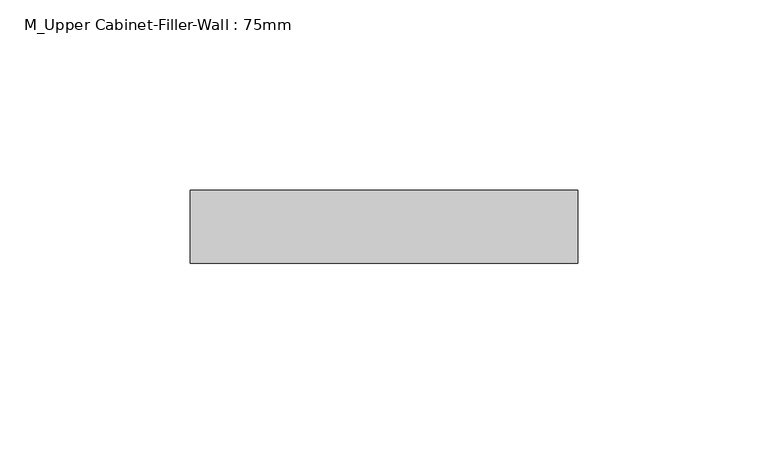
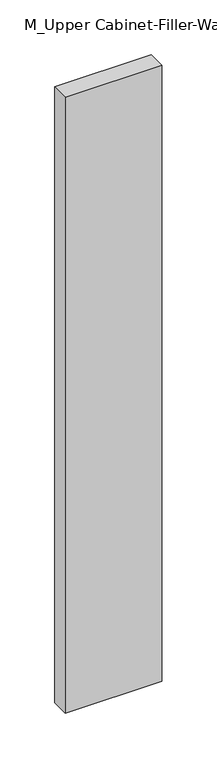
"""IFC4 building model written with IfcOpenShell, lengths in millimetres: furniture geometry, M_Upper Cabinet-Filler-Wall : 75mm."""

import ifcopenshell
import ifcopenshell.guid

model = None  # the IFC model being written
_history = None  # IfcOwnerHistory: only IFC2X3 demands one
_inside = {}  # id of a spatial element -> (the spatial element, [elements in it])
_under = {}  # id of a project, library or spatial element -> (it, [spatial elements below it])
_declared = {}  # id of a project -> (the project, [libraries it declares])
_typed = {}  # id of a type object -> (the type object, [elements of that type])
_made_of = {}  # id of a material, layer set ... -> (it, [elements and type objects made of it])


def new_model(schema):
    """Start an empty IFC model of exactly this schema.

    Asked for "IFC4X3", IfcOpenShell would pick the latest addendum, in which some entities
    have other attributes; the version numbers below select the first issue.
    IFC2X3 requires an IfcOwnerHistory on every rooted entity: one is made here for all.
    """
    global model, _history
    if schema == "IFC4X3":
        model = ifcopenshell.file(schema_version=(4, 3, 0, 0))
    else:
        model = ifcopenshell.file(schema=schema)
    _inside.clear()
    _under.clear()
    _declared.clear()
    _typed.clear()
    _made_of.clear()
    _history = None
    if model.schema == "IFC2X3":
        org = make("IfcOrganization", Name="unknown")
        user = make(
            "IfcPersonAndOrganization",
            ThePerson=make("IfcPerson", FamilyName="unknown"),
            TheOrganization=org,
        )
        app = make(
            "IfcApplication",
            ApplicationDeveloper=org,
            Version="unknown",
            ApplicationFullName="unknown",
            ApplicationIdentifier="unknown",
        )
        _history = make(
            "IfcOwnerHistory",
            OwningUser=user,
            OwningApplication=app,
            ChangeAction="ADDED",
            CreationDate=0,
        )
    return model


def make(cls, **values):
    """One entity of the class cls with the attributes given. An attribute that is None is left unset."""
    return model.create_entity(
        cls, **{name: value for name, value in values.items() if value is not None}
    )


def rooted(cls, **values):
    """An entity with a GlobalId (a new one), such as an element, a storey or a relation."""
    return make(cls, GlobalId=ifcopenshell.guid.new(), OwnerHistory=_history, **values)


def si_unit(unit_type, name, prefix=None):
    """IfcSIUnit, for example si_unit("LENGTHUNIT", "METRE", prefix="MILLI")."""
    return make("IfcSIUnit", UnitType=unit_type, Prefix=prefix, Name=name)


def assignment(units):
    """IfcUnitAssignment: the units of a project."""
    return None if units is None else make("IfcUnitAssignment", Units=units)


def point(xyz):
    """IfcCartesianPoint."""
    return None if xyz is None else make("IfcCartesianPoint", Coordinates=xyz)


def direction(xyz):
    """IfcDirection."""
    return None if xyz is None else make("IfcDirection", DirectionRatios=xyz)


def frame(location, z_axis=None, x_axis=None):
    """IfcAxis2Placement3D, a coordinate frame: its origin and axes. An axis left out is left unset."""
    return make(
        "IfcAxis2Placement3D",
        Location=point(location),
        Axis=direction(z_axis),
        RefDirection=direction(x_axis),
    )


def origin():
    """The frame at (0, 0, 0) with its axes left unset."""
    return frame((0.0, 0.0, 0.0))


def place(relative_to, where):
    """IfcLocalPlacement: puts the frame where relative to a parent placement (None: the world)."""
    return make(
        "IfcLocalPlacement", PlacementRelTo=relative_to, RelativePlacement=where
    )


def context(
    kind, dimensions, precision=None, world=None, true_north=None, identifier=None
):
    """IfcGeometricRepresentationContext, for example the 3D "Model" context."""
    return make(
        "IfcGeometricRepresentationContext",
        ContextIdentifier=identifier,
        ContextType=kind,
        CoordinateSpaceDimension=dimensions,
        Precision=precision,
        WorldCoordinateSystem=world,
        TrueNorth=true_north,
    )


def project(units=None, contexts=None):
    """IfcProject with its units and contexts."""
    return rooted(
        "IfcProject",
        Name="project",
        RepresentationContexts=contexts,
        UnitsInContext=assignment(units),
    )


def spatial(cls, under=None, at=None, **own):
    """A site, building, storey or space (cls), placed at a placement, below another one or the project."""
    s = rooted(cls, ObjectPlacement=at, **own)
    if under is not None:
        _under.setdefault(under.id(), (under, []))[1].append(s)
    return s


def polyline(points):
    """IfcPolyline through the points."""
    return make("IfcPolyline", Points=[point(p) for p in points])


def outline(outer, holes=None, kind="AREA"):
    """IfcArbitraryClosedProfileDef: a profile drawn as a closed curve; with holes, ...WithVoids."""
    if holes is None:
        return make("IfcArbitraryClosedProfileDef", ProfileType=kind, OuterCurve=outer)
    return make(
        "IfcArbitraryProfileDefWithVoids",
        ProfileType=kind,
        OuterCurve=outer,
        InnerCurves=holes,
    )


def extrude(swept, where, along, depth):
    """IfcExtrudedAreaSolid: the profile swept, set in the frame where, extruded along a direction by depth."""
    return make(
        "IfcExtrudedAreaSolid",
        SweptArea=swept,
        Position=where,
        ExtrudedDirection=direction(along),
        Depth=depth,
    )


def shape(context_of_items, identifier, shape_type, items):
    """IfcShapeRepresentation: the items that make up one representation, for example the "Body"."""
    return make(
        "IfcShapeRepresentation",
        ContextOfItems=context_of_items,
        RepresentationIdentifier=identifier,
        RepresentationType=shape_type,
        Items=items,
    )


def source(mapping_origin, context_of_items, identifier, shape_type, items):
    """IfcRepresentationMap: a shape defined once, which mapped items show again and again."""
    return make(
        "IfcRepresentationMap",
        MappingOrigin=mapping_origin,
        MappedRepresentation=shape(context_of_items, identifier, shape_type, items),
    )


def transform(
    local_origin,
    x_axis=None,
    y_axis=None,
    z_axis=None,
    scale=None,
    scale2=None,
    scale3=None,
    uniform=True,
):
    """IfcCartesianTransformationOperator3D, or its non-uniform kind. x_axis, y_axis, z_axis: its Axis1, 2, 3."""
    if uniform:
        return make(
            "IfcCartesianTransformationOperator3D",
            Axis1=direction(x_axis),
            Axis2=direction(y_axis),
            LocalOrigin=point(local_origin),
            Scale=scale,
            Axis3=direction(z_axis),
        )
    return make(
        "IfcCartesianTransformationOperator3DnonUniform",
        Axis1=direction(x_axis),
        Axis2=direction(y_axis),
        LocalOrigin=point(local_origin),
        Scale=scale,
        Axis3=direction(z_axis),
        Scale2=scale2,
        Scale3=scale3,
    )


def mapped(mapping_source, mapping_target):
    """IfcMappedItem: shows the shape of a source again, moved by a transform."""
    return make(
        "IfcMappedItem", MappingSource=mapping_source, MappingTarget=mapping_target
    )


def made_of(thing, what):
    """Note that an element or type object is made of a material, layer set ...; save() writes the relation."""
    if what is not None:
        _made_of.setdefault(what.id(), (what, []))[1].append(thing)
    return thing


def element(
    cls,
    number,
    at=None,
    inside=None,
    cuts=None,
    type_object=None,
    material=None,
    context=None,
    identifier="Body",
    shape_type=None,
    held_by="IfcProductDefinitionShape",
    body=None,
    shapes=None,
    **own,
):
    """One element of the class cls, such as IfcWall. Its Tag is "e" and its number.

    at: its placement. inside: the storey or other place that contains it. cuts: it is an
    opening in that element (IfcRelVoidsElement). A single representation is given by context,
    identifier, shape_type and body (its items); several are given by shapes. held_by: the class
    of the entity that holds the representations. save() writes the other relations.
    """
    e = rooted(cls, Tag="e%d" % number, ObjectPlacement=at, **own)
    if body is not None:
        shapes = [shape(context, identifier, shape_type, body)]
    if shapes is not None:
        e.Representation = make(held_by, Representations=shapes)
    if inside is not None:
        _inside.setdefault(inside.id(), (inside, []))[1].append(e)
    if cuts is not None:
        rooted(
            "IfcRelVoidsElement", RelatingBuildingElement=cuts, RelatedOpeningElement=e
        )
    if type_object is not None:
        _typed.setdefault(type_object.id(), (type_object, []))[1].append(e)
    return made_of(e, material)


def aggregate(whole, parts):
    """IfcRelAggregates: a whole, such as a stair, and the parts it consists of."""
    return rooted("IfcRelAggregates", RelatingObject=whole, RelatedObjects=parts)


def save(model, path):
    """Write the relations noted so far, then the file.

    IfcRelAggregates (storeys below a building ...), IfcRelContainedInSpatialStructure (elements
    in a storey), IfcRelDefinesByType, IfcRelAssociatesMaterial and IfcRelDeclares: one each for
    every whole, place, type object, material and project.
    """
    for whole, parts in _under.values():
        aggregate(whole, parts)
    for where, things in _inside.values():
        rooted(
            "IfcRelContainedInSpatialStructure",
            RelatedElements=things,
            RelatingStructure=where,
        )
    for kind, things in _typed.values():
        rooted("IfcRelDefinesByType", RelatedObjects=things, RelatingType=kind)
    for what, things in _made_of.values():
        rooted("IfcRelAssociatesMaterial", RelatedObjects=things, RelatingMaterial=what)
    for by, libraries in _declared.values():
        rooted("IfcRelDeclares", RelatingContext=by, RelatedDefinitions=libraries)
    model.write(path)


def m_upper_cabinet_filler_wall_75mm_90d919fc(model_context):
    return source(origin(), model_context, "Body", "SweptSolid", [
        extrude(outline(polyline([(-21.0288372, 38.1), (-21.0288372, 57.15), (80.5711628, 57.15), (80.5711628, 38.1), (-21.0288372, 38.1)])), frame((0.0, 0.0, 1314.2), z_axis=(0.0, 0.0, 1.0), x_axis=(1.0, 0.0, 0.0)), (0.0, 0.0, 1.0), 685.8),
    ])


if __name__ == "__main__":
    model = new_model("IFC4")
    model_context = context("Model", 3, world=origin())
    ifc_project = project(units=[si_unit("LENGTHUNIT", "METRE", prefix="MILLI")], contexts=[model_context])
    site = spatial("IfcSite", under=ifc_project)
    building = spatial("IfcBuilding", under=site)
    placement = place(None, origin())
    m_upper_cabinet_filler_wall_75mm_shape = m_upper_cabinet_filler_wall_75mm_90d919fc(model_context)
    element("IfcFurniture", 1, ObjectType="M_Upper Cabinet-Filler-Wall : 75mm", at=placement, inside=building, context=model_context, shape_type="MappedRepresentation", body=[
        mapped(m_upper_cabinet_filler_wall_75mm_shape, transform((0.0, 0.0, 0.0), x_axis=(1.0, 0.0, 0.0), y_axis=(0.0, 1.0, 0.0), z_axis=(0.0, 0.0, 1.0))),
    ])
    save(model, "model.ifc")

# Revit data of these elements
# Type "M_Upper Cabinet-Filler-Wall : 75mm"
#   Depth = 0' - 1"
#   Height = 2' - 3"
#   Top Of Cabinet = 6' - 6.74016"
#   Width = 0' - 4"
#   Cabinet Material = none
#   Default Elevation = 0
# Element 1 (IfcFurniture, "M_Upper Cabinet-Filler-Wall : 75mm")
#   Materials on its faces: "Cabinets"
# Materials
#   "Cabinets": class "Miscellaneous", colour RGB 249 249 249, transparency 0
